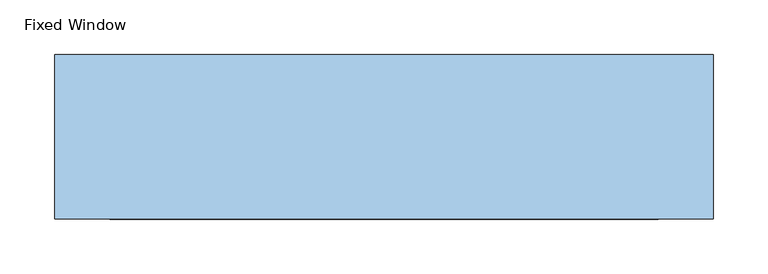
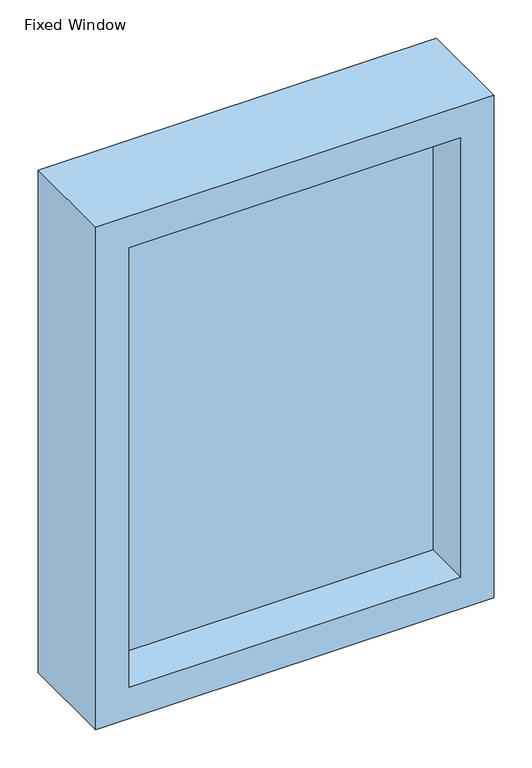
"""IFC4 building model written with IfcOpenShell, lengths in millimetres: window geometry, Fixed Window : H_WD_AMW_AL Window_DG_W600xH600_Fixed_1H1V."""

from ifc_helpers import new_model, si_unit, frame, origin, place, context, project, spatial, polyline, outline, extrude, source, transform, mapped, element, save


def fixed_window_37dd25d6(model_context):
    return source(origin(), model_context, "Body", "SweptSolid", [
        extrude(outline(polyline([(-250.0, 3.0), (250.0, 3.0), (250.0, -3.0), (-250.0, -3.0), (-250.0, 3.0)])), frame((0.0, 0.0, 850.0), z_axis=(0.0, 0.0, 1.0), x_axis=(1.0, 0.0, 0.0)), (0.0, 0.0, 1.0), 700.0),
        extrude(outline(polyline([(1600.0, -300.0), (800.0, -300.0), (800.0, 300.0), (1600.0, 300.0), (1600.0, -300.0)]), holes=[polyline([(1550.0, -250.0), (1550.0, 250.0), (850.0, 250.0), (850.0, -250.0), (1550.0, -250.0)])]), frame((0.0, -75.0, 0.0), z_axis=(0.0, 1.0, 0.0), x_axis=(0.0, 0.0, 1.0)), (0.0, 0.0, 1.0), 150.0),
    ])


if __name__ == "__main__":
    model = new_model("IFC4")
    model_context = context("Model", 3, world=origin())
    ifc_project = project(units=[si_unit("LENGTHUNIT", "METRE", prefix="MILLI")], contexts=[model_context])
    site = spatial("IfcSite", under=ifc_project)
    building = spatial("IfcBuilding", under=site)
    placement = place(None, origin())
    fixed_window_shape = fixed_window_37dd25d6(model_context)
    element("IfcWindow", 1, ObjectType="Fixed Window : H_WD_AMW_AL Window_DG_W600xH600_Fixed_1H1V", at=placement, inside=building, context=model_context, shape_type="MappedRepresentation", body=[
        mapped(fixed_window_shape, transform((0.0, 0.0, 0.0), x_axis=(1.0, 0.0, 0.0), y_axis=(0.0, 1.0, 0.0), z_axis=(0.0, 0.0, 1.0))),
    ])
    save(model, "model.ifc")

# Revit data of these elements
# Type "Fixed Window : H_WD_AMW_AL Window_DG_W600xH600_Fixed_1H1V"
#   Type Mark = "AW"
#   Analytic Construction = "<None>"
#   창 두께 = 0.1500 m
#   Height = 0.8000 m
#   절반 창 두께 = 0.0750 m
#   기본 씰 높이 = 0.8000 m
#   Width = 0.6000 m
#   Define Thermal Properties by = 1
#   창 패널 = AW2 창 패널
#   창 프레임 = A04AQ127-00002_Aluminum Window_None FP
#   Wall Closure = (empty or 0)
# Element 1 (IfcWindow, "Fixed Window : H_WD_AMW_AL Window_DG_W600xH600_Fixed_1H1V")
#   Materials on its faces: "A04AQ127-00002_Aluminum Window_None FP", "AW2 창 패널"
# Materials
#   "AW2 창 패널": class "유리", colour RGB 0 0 255, transparency 0.75
#   "A04AQ127-00002_Aluminum Window_None FP": class "금속", colour RGB 247 247 247, transparency 0, Cost = 0
